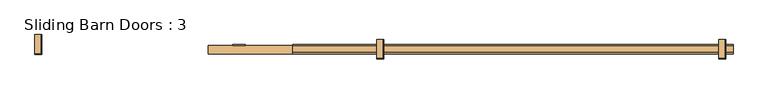
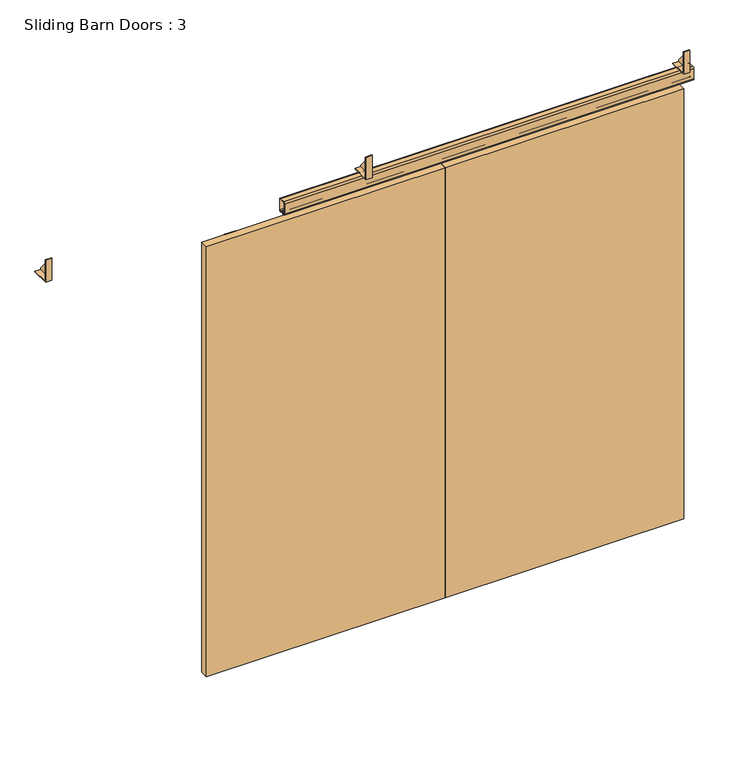
"""IFC4 building model written with IfcOpenShell, lengths in millimetres: door geometry, Sliding Barn Doors : 3."""

from ifc_helpers import new_model, si_unit, point, frame, frame_2d, origin, place, context, project, spatial, polyline, circle_curve, trimmed, segment, composite_curve, outline, extrude, source, transform, mapped, element, save


def sliding_barn_doors_3_ff6fe0db(model_context):
    return source(origin(), model_context, "Body", "SweptSolid", [
        extrude(outline(polyline([(158.75, 2152.65), (158.75, 2146.3), (79.375, 2146.3), (79.375, 2247.773), (158.75, 2152.65)])), frame((-1635.1746094, 0.0, 0.0), z_axis=(1.0, 0.0, 0.0), x_axis=(0.0, 1.0, 0.0)), (0.0, 0.0, 1.0), 3.175),
        extrude(outline(polyline([(76.2, 2143.125), (76.2, 2247.773), (79.375, 2247.773), (79.375, 2146.3), (158.75, 2146.3), (158.75, 2143.125), (76.2, 2143.125)])), frame((-1660.4753906, 0.0, 0.0), z_axis=(1.0, 0.0, 0.0), x_axis=(0.0, 1.0, 0.0)), (0.0, 0.0, 1.0), 28.4757812),
        extrude(outline(polyline([(139.7, 2152.65), (139.7, 2146.3), (60.325, 2146.3), (60.325, 2247.773), (139.7, 2152.65)])), frame((-215.1558594, 0.0, 0.0), z_axis=(1.0, 0.0, 0.0), x_axis=(0.0, 1.0, 0.0)), (0.0, 0.0, 1.0), 3.175),
        extrude(outline(polyline([(57.15, 2143.125), (57.15, 2247.773), (60.325, 2247.773), (60.325, 2146.3), (139.7, 2146.3), (139.7, 2143.125), (57.15, 2143.125)])), frame((-240.4566406, 0.0, 0.0), z_axis=(1.0, 0.0, 0.0), x_axis=(0.0, 1.0, 0.0)), (0.0, 0.0, 1.0), 28.4757812),
        extrude(outline(polyline([(139.7, 2152.65), (139.7, 2146.3), (60.325, 2146.3), (60.325, 2247.773), (139.7, 2152.65)])), frame((1204.8628906, 0.0, 0.0), z_axis=(1.0, 0.0, 0.0), x_axis=(0.0, 1.0, 0.0)), (0.0, 0.0, 1.0), 3.175),
        extrude(outline(polyline([(57.15, 2143.125), (57.15, 2247.773), (60.325, 2247.773), (60.325, 2146.3), (139.7, 2146.3), (139.7, 2143.125), (57.15, 2143.125)])), frame((1179.5621094, 0.0, 0.0), z_axis=(1.0, 0.0, 0.0), x_axis=(0.0, 1.0, 0.0)), (0.0, 0.0, 1.0), 28.4757812),
        extrude(outline(polyline([(-838.454, 117.475), (-787.146, 117.475), (-787.146, 114.3), (-838.454, 114.3), (-838.454, 117.475)])), frame((0.0, 0.0, 1889.252), z_axis=(0.0, 0.0, 1.0), x_axis=(1.0, 0.0, 0.0)), (0.0, 0.0, 1.0), 168.148),
        extrude(outline(polyline([(-25.654, 117.475), (25.654, 117.475), (25.654, 114.3), (-25.654, 114.3), (-25.654, 117.475)])), frame((0.0, 0.0, 1889.252), z_axis=(0.0, 0.0, 1.0), x_axis=(1.0, 0.0, 0.0)), (0.0, 0.0, 1.0), 168.148),
        extrude(outline(polyline([(228.346, 117.475), (279.654, 117.475), (279.654, 114.3), (228.346, 114.3), (228.346, 117.475)])), frame((0.0, 0.0, 1889.252), z_axis=(0.0, 0.0, 1.0), x_axis=(1.0, 0.0, 0.0)), (0.0, 0.0, 1.0), 168.148),
        extrude(outline(polyline([(1041.146, 117.475), (1092.454, 117.475), (1092.454, 114.3), (1041.146, 114.3), (1041.146, 117.475)])), frame((0.0, 0.0, 1889.252), z_axis=(0.0, 0.0, 1.0), x_axis=(1.0, 0.0, 0.0)), (0.0, 0.0, 1.0), 168.148),
        extrude(outline(polyline([(-939.8, 114.3), (127.0, 114.3), (127.0, 79.375), (-939.8, 79.375), (-939.8, 114.3)])), frame((0.0, 0.0, 25.4), z_axis=(0.0, 0.0, 1.0), x_axis=(1.0, 0.0, 0.0)), (0.0, 0.0, 1.0), 2032.0),
        extrude(outline(polyline([(127.0, 114.3), (1193.8, 114.3), (1193.8, 79.375), (127.0, 79.375), (127.0, 114.3)])), frame((0.0, 0.0, 25.4), z_axis=(0.0, 0.0, 1.0), x_axis=(1.0, 0.0, 0.0)), (0.0, 0.0, 1.0), 2032.0),
        extrude(outline(composite_curve([segment(polyline([(85.725, 2143.125), (111.252, 2143.125)]), True, "CONTINUOUS"), segment(trimmed(circle_curve(frame_2d((111.252, 2136.775)), 6.35), [point((111.252, 2143.125))], [point((117.602, 2136.775))], False, "CARTESIAN"), True, "CONTINUOUS"), segment(polyline([(117.602, 2136.775), (117.602, 2088.515)]), True, "CONTINUOUS"), segment(trimmed(circle_curve(frame_2d((111.252, 2088.515)), 6.35), [point((117.602, 2088.515))], [point((111.252, 2082.165))], False, "CARTESIAN"), True, "CONTINUOUS"), segment(polyline([(111.252, 2082.165), (105.8433147, 2082.165)]), True, "CONTINUOUS"), segment(trimmed(circle_curve(frame_2d((105.8433147, 2083.7525)), 1.5875), [point((105.8433147, 2082.165))], [point((104.2849816, 2083.4495907))], False, "CARTESIAN"), True, "CONTINUOUS"), segment(polyline([(104.2849816, 2083.4495907), (102.8594659, 2090.7832331), (104.3756029, 2090.7832331), (105.7615251, 2083.6532812), (111.252, 2083.6532812)]), True, "CONTINUOUS"), segment(trimmed(circle_curve(frame_2d((111.252, 2088.515)), 4.8617187), [point((111.252, 2083.6532812))], [point((116.1137188, 2088.515))], True, "CARTESIAN"), True, "CONTINUOUS"), segment(polyline([(116.1137188, 2088.515), (116.1137188, 2136.775)]), True, "CONTINUOUS"), segment(trimmed(circle_curve(frame_2d((111.252, 2136.775)), 4.8617187), [point((116.1137188, 2136.775))], [point((111.252, 2141.6367187))], True, "CARTESIAN"), True, "CONTINUOUS"), segment(polyline([(111.252, 2141.6367187), (85.725, 2141.6367187)]), True, "CONTINUOUS"), segment(trimmed(circle_curve(frame_2d((85.725, 2136.775)), 4.8617187), [point((85.725, 2141.6367187))], [point((80.8632813, 2136.775))], True, "CARTESIAN"), True, "CONTINUOUS"), segment(polyline([(80.8632813, 2136.775), (80.8632813, 2088.515)]), True, "CONTINUOUS"), segment(trimmed(circle_curve(frame_2d((85.725, 2088.515)), 4.8617187), [point((80.8632813, 2088.515))], [point((85.725, 2083.6532812))], True, "CARTESIAN"), True, "CONTINUOUS"), segment(polyline([(85.725, 2083.6532812), (91.2154749, 2083.6532812), (92.6013971, 2090.7832331), (94.1175341, 2090.7832331), (92.6920184, 2083.4495907)]), True, "CONTINUOUS"), segment(trimmed(circle_curve(frame_2d((91.1336853, 2083.7525)), 1.5875), [point((92.6920184, 2083.4495907))], [point((91.1336853, 2082.165))], False, "CARTESIAN"), True, "CONTINUOUS"), segment(polyline([(91.1336853, 2082.165), (85.725, 2082.165)]), True, "CONTINUOUS"), segment(trimmed(circle_curve(frame_2d((85.725, 2088.515)), 6.35), [point((85.725, 2082.165))], [point((79.375, 2088.515))], False, "CARTESIAN"), True, "CONTINUOUS"), segment(polyline([(79.375, 2088.515), (79.375, 2136.775)]), True, "CONTINUOUS"), segment(trimmed(circle_curve(frame_2d((85.725, 2136.775)), 6.35), [point((79.375, 2136.775))], [point((85.725, 2143.125))], False, "CARTESIAN"), True, "CONTINUOUS")], self_intersect=False)), frame((-590.55, 0.0, 0.0), z_axis=(1.0, 0.0, 0.0), x_axis=(0.0, 1.0, 0.0)), (0.0, 0.0, 1.0), 1828.8),
    ])


if __name__ == "__main__":
    model = new_model("IFC4")
    model_context = context("Model", 3, world=origin())
    ifc_project = project(units=[si_unit("LENGTHUNIT", "METRE", prefix="MILLI")], contexts=[model_context])
    site = spatial("IfcSite", under=ifc_project)
    building = spatial("IfcBuilding", under=site)
    placement = place(None, origin())
    sliding_barn_doors_3_shape = sliding_barn_doors_3_ff6fe0db(model_context)
    element("IfcDoor", 1, ObjectType="Sliding Barn Doors : 3", at=placement, inside=building, context=model_context, shape_type="MappedRepresentation", body=[
        mapped(sliding_barn_doors_3_shape, transform((0.0, 0.0, 0.0), x_axis=(1.0, 0.0, 0.0), y_axis=(0.0, 1.0, 0.0), z_axis=(0.0, 0.0, 1.0))),
    ])
    save(model, "model.ifc")

# Revit data of these elements
# Type "Sliding Barn Doors : 3"
#   Type Mark = "43"
#   OD_DS_Door_Type = "SLIDER"
#   Analytic Construction = "<None>"
#   rail_overlap_left = 0' - 3 3/4"
#   rail_length = 6' - 0"
#   overlap_left = 0' - 2"
#   overlap = 0' - 0"
#   bracket_right = 1' - 7 13/16"
#   bracket_left = 0' - 2"
#   Thickness = 0' - 1 3/8"
#   Panel Width = 3' - 6"
#   Panel Height = 6' - 8"
#   Gap 2 = 0' - 0 1/2"
#   Gap 1 = 0' - 0 7/8"
#   Frame Projection Ext. = 0' - 1"
#   Frame Projection Int. = 0' - 1"
#   Frame Width = 0' - 3"
#   Height = 6' - 5 3/8"
#   Width = 7' - 6"
#   Bracket_offset = 0' - 5"
#   Door_4 = no
#   Door_3 = no
#   Hardware Material = Metal - Aluminum
#   Door Material = Closet_1
#   Function = (empty or 0)
#   Wall Closure = (empty or 0)
# Element 1 (IfcDoor, "Sliding Barn Doors : 3")
#   Materials on its faces: "Metal - Aluminum", "Closet_1"
# Materials
#   "Metal - Aluminum": class "Metal", colour RGB 247 247 247, transparency 0
#   "Closet_1": class "Paint", colour RGB 200 194 183, transparency 0, Cost = 0
